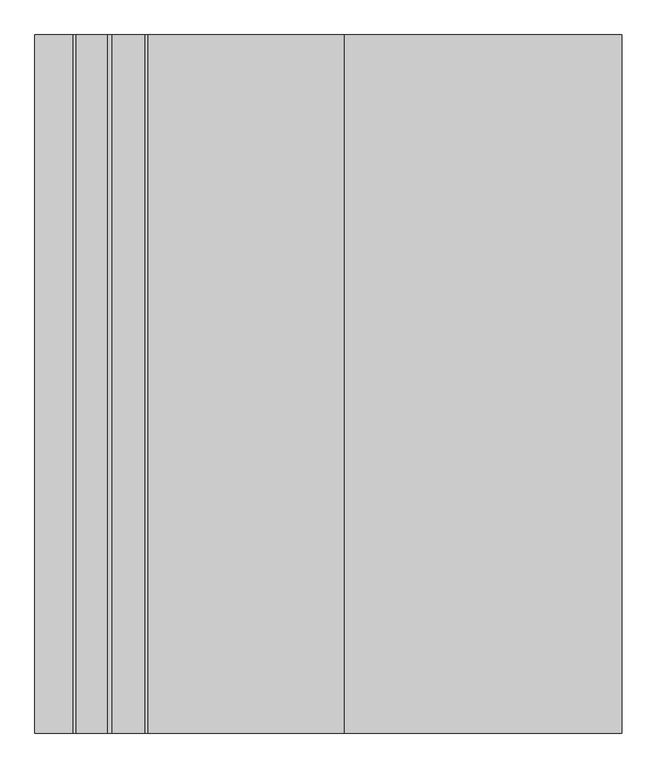
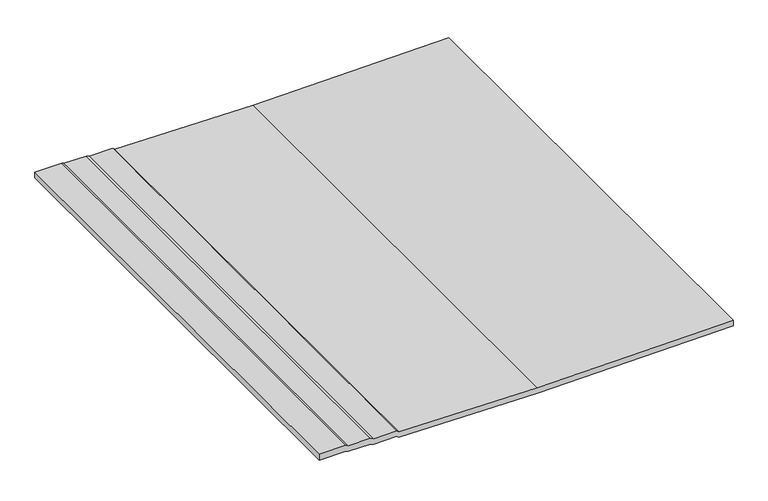
"""IFC4 building model written with IfcOpenShell, lengths in millimetres: proxy geometry, GRAVEL BALLAST002 4284 : GRAVEL BALLAST002 4284."""

import ifcopenshell
import ifcopenshell.guid

model = None  # the IFC model being written
_history = None  # IfcOwnerHistory: only IFC2X3 demands one
_inside = {}  # id of a spatial element -> (the spatial element, [elements in it])
_under = {}  # id of a project, library or spatial element -> (it, [spatial elements below it])
_declared = {}  # id of a project -> (the project, [libraries it declares])
_typed = {}  # id of a type object -> (the type object, [elements of that type])
_made_of = {}  # id of a material, layer set ... -> (it, [elements and type objects made of it])


def new_model(schema):
    """Start an empty IFC model of exactly this schema.

    Asked for "IFC4X3", IfcOpenShell would pick the latest addendum, in which some entities
    have other attributes; the version numbers below select the first issue.
    IFC2X3 requires an IfcOwnerHistory on every rooted entity: one is made here for all.
    """
    global model, _history
    if schema == "IFC4X3":
        model = ifcopenshell.file(schema_version=(4, 3, 0, 0))
    else:
        model = ifcopenshell.file(schema=schema)
    _inside.clear()
    _under.clear()
    _declared.clear()
    _typed.clear()
    _made_of.clear()
    _history = None
    if model.schema == "IFC2X3":
        org = make("IfcOrganization", Name="unknown")
        user = make(
            "IfcPersonAndOrganization",
            ThePerson=make("IfcPerson", FamilyName="unknown"),
            TheOrganization=org,
        )
        app = make(
            "IfcApplication",
            ApplicationDeveloper=org,
            Version="unknown",
            ApplicationFullName="unknown",
            ApplicationIdentifier="unknown",
        )
        _history = make(
            "IfcOwnerHistory",
            OwningUser=user,
            OwningApplication=app,
            ChangeAction="ADDED",
            CreationDate=0,
        )
    return model


def make(cls, **values):
    """One entity of the class cls with the attributes given. An attribute that is None is left unset."""
    return model.create_entity(
        cls, **{name: value for name, value in values.items() if value is not None}
    )


def rooted(cls, **values):
    """An entity with a GlobalId (a new one), such as an element, a storey or a relation."""
    return make(cls, GlobalId=ifcopenshell.guid.new(), OwnerHistory=_history, **values)


def si_unit(unit_type, name, prefix=None):
    """IfcSIUnit, for example si_unit("LENGTHUNIT", "METRE", prefix="MILLI")."""
    return make("IfcSIUnit", UnitType=unit_type, Prefix=prefix, Name=name)


def assignment(units):
    """IfcUnitAssignment: the units of a project."""
    return None if units is None else make("IfcUnitAssignment", Units=units)


def point(xyz):
    """IfcCartesianPoint."""
    return None if xyz is None else make("IfcCartesianPoint", Coordinates=xyz)


def direction(xyz):
    """IfcDirection."""
    return None if xyz is None else make("IfcDirection", DirectionRatios=xyz)


def frame(location, z_axis=None, x_axis=None):
    """IfcAxis2Placement3D, a coordinate frame: its origin and axes. An axis left out is left unset."""
    return make(
        "IfcAxis2Placement3D",
        Location=point(location),
        Axis=direction(z_axis),
        RefDirection=direction(x_axis),
    )


def origin():
    """The frame at (0, 0, 0) with its axes left unset."""
    return frame((0.0, 0.0, 0.0))


def place(relative_to, where):
    """IfcLocalPlacement: puts the frame where relative to a parent placement (None: the world)."""
    return make(
        "IfcLocalPlacement", PlacementRelTo=relative_to, RelativePlacement=where
    )


def context(
    kind, dimensions, precision=None, world=None, true_north=None, identifier=None
):
    """IfcGeometricRepresentationContext, for example the 3D "Model" context."""
    return make(
        "IfcGeometricRepresentationContext",
        ContextIdentifier=identifier,
        ContextType=kind,
        CoordinateSpaceDimension=dimensions,
        Precision=precision,
        WorldCoordinateSystem=world,
        TrueNorth=true_north,
    )


def project(units=None, contexts=None):
    """IfcProject with its units and contexts."""
    return rooted(
        "IfcProject",
        Name="project",
        RepresentationContexts=contexts,
        UnitsInContext=assignment(units),
    )


def spatial(cls, under=None, at=None, **own):
    """A site, building, storey or space (cls), placed at a placement, below another one or the project."""
    s = rooted(cls, ObjectPlacement=at, **own)
    if under is not None:
        _under.setdefault(under.id(), (under, []))[1].append(s)
    return s


def polyline(points):
    """IfcPolyline through the points."""
    return make("IfcPolyline", Points=[point(p) for p in points])


def outline(outer, holes=None, kind="AREA"):
    """IfcArbitraryClosedProfileDef: a profile drawn as a closed curve; with holes, ...WithVoids."""
    if holes is None:
        return make("IfcArbitraryClosedProfileDef", ProfileType=kind, OuterCurve=outer)
    return make(
        "IfcArbitraryProfileDefWithVoids",
        ProfileType=kind,
        OuterCurve=outer,
        InnerCurves=holes,
    )


def extrude(swept, where, along, depth):
    """IfcExtrudedAreaSolid: the profile swept, set in the frame where, extruded along a direction by depth."""
    return make(
        "IfcExtrudedAreaSolid",
        SweptArea=swept,
        Position=where,
        ExtrudedDirection=direction(along),
        Depth=depth,
    )


def shape(context_of_items, identifier, shape_type, items):
    """IfcShapeRepresentation: the items that make up one representation, for example the "Body"."""
    return make(
        "IfcShapeRepresentation",
        ContextOfItems=context_of_items,
        RepresentationIdentifier=identifier,
        RepresentationType=shape_type,
        Items=items,
    )


def source(mapping_origin, context_of_items, identifier, shape_type, items):
    """IfcRepresentationMap: a shape defined once, which mapped items show again and again."""
    return make(
        "IfcRepresentationMap",
        MappingOrigin=mapping_origin,
        MappedRepresentation=shape(context_of_items, identifier, shape_type, items),
    )


def transform(
    local_origin,
    x_axis=None,
    y_axis=None,
    z_axis=None,
    scale=None,
    scale2=None,
    scale3=None,
    uniform=True,
):
    """IfcCartesianTransformationOperator3D, or its non-uniform kind. x_axis, y_axis, z_axis: its Axis1, 2, 3."""
    if uniform:
        return make(
            "IfcCartesianTransformationOperator3D",
            Axis1=direction(x_axis),
            Axis2=direction(y_axis),
            LocalOrigin=point(local_origin),
            Scale=scale,
            Axis3=direction(z_axis),
        )
    return make(
        "IfcCartesianTransformationOperator3DnonUniform",
        Axis1=direction(x_axis),
        Axis2=direction(y_axis),
        LocalOrigin=point(local_origin),
        Scale=scale,
        Axis3=direction(z_axis),
        Scale2=scale2,
        Scale3=scale3,
    )


def mapped(mapping_source, mapping_target):
    """IfcMappedItem: shows the shape of a source again, moved by a transform."""
    return make(
        "IfcMappedItem", MappingSource=mapping_source, MappingTarget=mapping_target
    )


def made_of(thing, what):
    """Note that an element or type object is made of a material, layer set ...; save() writes the relation."""
    if what is not None:
        _made_of.setdefault(what.id(), (what, []))[1].append(thing)
    return thing


def element(
    cls,
    number,
    at=None,
    inside=None,
    cuts=None,
    type_object=None,
    material=None,
    context=None,
    identifier="Body",
    shape_type=None,
    held_by="IfcProductDefinitionShape",
    body=None,
    shapes=None,
    **own,
):
    """One element of the class cls, such as IfcWall. Its Tag is "e" and its number.

    at: its placement. inside: the storey or other place that contains it. cuts: it is an
    opening in that element (IfcRelVoidsElement). A single representation is given by context,
    identifier, shape_type and body (its items); several are given by shapes. held_by: the class
    of the entity that holds the representations. save() writes the other relations.
    """
    e = rooted(cls, Tag="e%d" % number, ObjectPlacement=at, **own)
    if body is not None:
        shapes = [shape(context, identifier, shape_type, body)]
    if shapes is not None:
        e.Representation = make(held_by, Representations=shapes)
    if inside is not None:
        _inside.setdefault(inside.id(), (inside, []))[1].append(e)
    if cuts is not None:
        rooted(
            "IfcRelVoidsElement", RelatingBuildingElement=cuts, RelatedOpeningElement=e
        )
    if type_object is not None:
        _typed.setdefault(type_object.id(), (type_object, []))[1].append(e)
    return made_of(e, material)


def aggregate(whole, parts):
    """IfcRelAggregates: a whole, such as a stair, and the parts it consists of."""
    return rooted("IfcRelAggregates", RelatingObject=whole, RelatedObjects=parts)


def save(model, path):
    """Write the relations noted so far, then the file.

    IfcRelAggregates (storeys below a building ...), IfcRelContainedInSpatialStructure (elements
    in a storey), IfcRelDefinesByType, IfcRelAssociatesMaterial and IfcRelDeclares: one each for
    every whole, place, type object, material and project.
    """
    for whole, parts in _under.values():
        aggregate(whole, parts)
    for where, things in _inside.values():
        rooted(
            "IfcRelContainedInSpatialStructure",
            RelatedElements=things,
            RelatingStructure=where,
        )
    for kind, things in _typed.values():
        rooted("IfcRelDefinesByType", RelatedObjects=things, RelatingType=kind)
    for what, things in _made_of.values():
        rooted("IfcRelAssociatesMaterial", RelatedObjects=things, RelatingMaterial=what)
    for by, libraries in _declared.values():
        rooted("IfcRelDeclares", RelatingContext=by, RelatedDefinitions=libraries)
    model.write(path)


def generic_models_70855ca7(model_context):
    return source(origin(), model_context, "Body", "SweptSolid", [
        extrude(outline(polyline([(40274.2359465, -2672.3662777), (40269.9546965, -2663.6558285), (40269.9546965, -2573.0689144), (40264.2272344, -2560.2242751), (40265.8726651, -2466.2725277), (40258.4625089, -2457.9990902), (40250.2437589, -1894.9286556), (40261.546875, -1099.1907959), (40286.2851563, -1099.1907959), (40274.9820403, -1894.9286556), (40283.2007903, -2457.9990902), (40290.6109465, -2466.2725277), (40288.9655158, -2560.2242751), (40294.6929777, -2573.0689144), (40294.6929777, -2663.6558285), (40298.9742278, -2672.3662777), (40298.9742278, -2781.8657894), (40274.2359465, -2781.8657894), (40274.2359465, -2672.3662777)])), frame((0.0, -1052.6406573, 0.0), z_axis=(0.0, 1.0, 0.0), x_axis=(0.0, 0.0, 1.0)), (0.0, 0.0, 1.0), 2000.0),
    ])


if __name__ == "__main__":
    model = new_model("IFC4")
    model_context = context("Model", 3, world=origin())
    ifc_project = project(units=[si_unit("LENGTHUNIT", "METRE", prefix="MILLI")], contexts=[model_context])
    site = spatial("IfcSite", under=ifc_project)
    building = spatial("IfcBuilding", under=site)
    placement = place(None, origin())
    generic_models_shape = generic_models_70855ca7(model_context)
    element("IfcBuildingElementProxy", 1, Name="GRAVEL BALLAST002 4284 : GRAVEL BALLAST002 4284", ObjectType="GRAVEL BALLAST002 4284 : GRAVEL BALLAST002 4284", at=placement, inside=building, context=model_context, shape_type="MappedRepresentation", body=[
        mapped(generic_models_shape, transform((0.0, 0.0, 0.0), x_axis=(1.0, 0.0, 0.0), y_axis=(0.0, 1.0, 0.0), z_axis=(0.0, 0.0, 1.0))),
    ])
    save(model, "model.ifc")

# Revit data of these elements
# Type "GRAVEL BALLAST002 4284 : GRAVEL BALLAST002 4284"
#   NameOverride = "GRAVEL BALLAST002"
# Element 1 (IfcBuildingElementProxy, "GRAVEL BALLAST002 4284 : GRAVEL BALLAST002 4284")
#   Materials on its faces: "GRAVEL BALLAST"
# Materials
#   "GRAVEL BALLAST": class "Unassigned", colour RGB 128 128 128, transparency 0, Cost = 0
